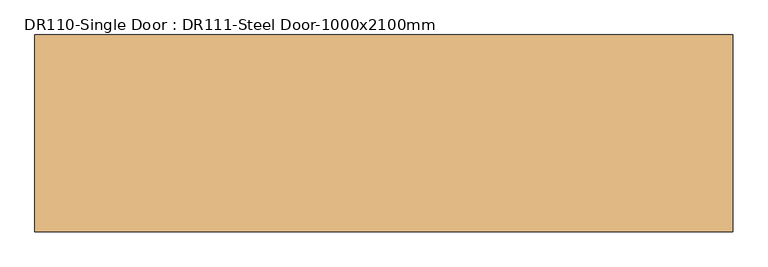
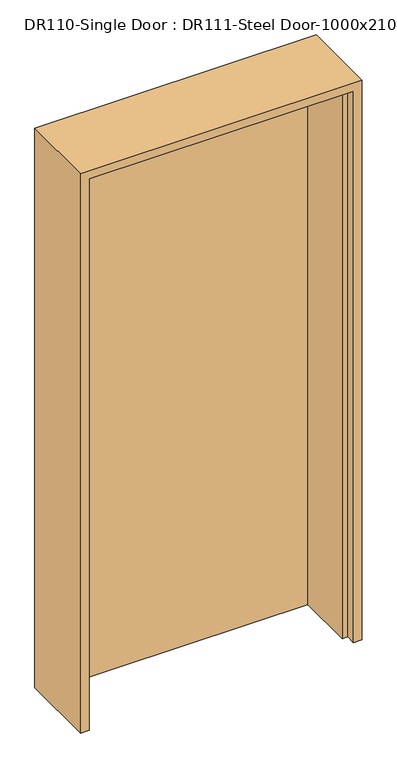
"""IFC4 building model written with IfcOpenShell, lengths in millimetres: door geometry, DR110-Single Door : DR111-Steel Door-1000x2100mm."""

import ifcopenshell
import ifcopenshell.guid

model = None  # the IFC model being written
_history = None  # IfcOwnerHistory: only IFC2X3 demands one
_inside = {}  # id of a spatial element -> (the spatial element, [elements in it])
_under = {}  # id of a project, library or spatial element -> (it, [spatial elements below it])
_declared = {}  # id of a project -> (the project, [libraries it declares])
_typed = {}  # id of a type object -> (the type object, [elements of that type])
_made_of = {}  # id of a material, layer set ... -> (it, [elements and type objects made of it])


def new_model(schema):
    """Start an empty IFC model of exactly this schema.

    Asked for "IFC4X3", IfcOpenShell would pick the latest addendum, in which some entities
    have other attributes; the version numbers below select the first issue.
    IFC2X3 requires an IfcOwnerHistory on every rooted entity: one is made here for all.
    """
    global model, _history
    if schema == "IFC4X3":
        model = ifcopenshell.file(schema_version=(4, 3, 0, 0))
    else:
        model = ifcopenshell.file(schema=schema)
    _inside.clear()
    _under.clear()
    _declared.clear()
    _typed.clear()
    _made_of.clear()
    _history = None
    if model.schema == "IFC2X3":
        org = make("IfcOrganization", Name="unknown")
        user = make(
            "IfcPersonAndOrganization",
            ThePerson=make("IfcPerson", FamilyName="unknown"),
            TheOrganization=org,
        )
        app = make(
            "IfcApplication",
            ApplicationDeveloper=org,
            Version="unknown",
            ApplicationFullName="unknown",
            ApplicationIdentifier="unknown",
        )
        _history = make(
            "IfcOwnerHistory",
            OwningUser=user,
            OwningApplication=app,
            ChangeAction="ADDED",
            CreationDate=0,
        )
    return model


def make(cls, **values):
    """One entity of the class cls with the attributes given. An attribute that is None is left unset."""
    return model.create_entity(
        cls, **{name: value for name, value in values.items() if value is not None}
    )


def rooted(cls, **values):
    """An entity with a GlobalId (a new one), such as an element, a storey or a relation."""
    return make(cls, GlobalId=ifcopenshell.guid.new(), OwnerHistory=_history, **values)


def si_unit(unit_type, name, prefix=None):
    """IfcSIUnit, for example si_unit("LENGTHUNIT", "METRE", prefix="MILLI")."""
    return make("IfcSIUnit", UnitType=unit_type, Prefix=prefix, Name=name)


def assignment(units):
    """IfcUnitAssignment: the units of a project."""
    return None if units is None else make("IfcUnitAssignment", Units=units)


def point(xyz):
    """IfcCartesianPoint."""
    return None if xyz is None else make("IfcCartesianPoint", Coordinates=xyz)


def direction(xyz):
    """IfcDirection."""
    return None if xyz is None else make("IfcDirection", DirectionRatios=xyz)


def frame(location, z_axis=None, x_axis=None):
    """IfcAxis2Placement3D, a coordinate frame: its origin and axes. An axis left out is left unset."""
    return make(
        "IfcAxis2Placement3D",
        Location=point(location),
        Axis=direction(z_axis),
        RefDirection=direction(x_axis),
    )


def origin():
    """The frame at (0, 0, 0) with its axes left unset."""
    return frame((0.0, 0.0, 0.0))


def origin_with_axes():
    """The frame at (0, 0, 0) with the z axis (0, 0, 1) and the x axis (1, 0, 0) written out."""
    return frame((0.0, 0.0, 0.0), z_axis=(0.0, 0.0, 1.0), x_axis=(1.0, 0.0, 0.0))


def place(relative_to, where):
    """IfcLocalPlacement: puts the frame where relative to a parent placement (None: the world)."""
    return make(
        "IfcLocalPlacement", PlacementRelTo=relative_to, RelativePlacement=where
    )


def context(
    kind, dimensions, precision=None, world=None, true_north=None, identifier=None
):
    """IfcGeometricRepresentationContext, for example the 3D "Model" context."""
    return make(
        "IfcGeometricRepresentationContext",
        ContextIdentifier=identifier,
        ContextType=kind,
        CoordinateSpaceDimension=dimensions,
        Precision=precision,
        WorldCoordinateSystem=world,
        TrueNorth=true_north,
    )


def project(units=None, contexts=None):
    """IfcProject with its units and contexts."""
    return rooted(
        "IfcProject",
        Name="project",
        RepresentationContexts=contexts,
        UnitsInContext=assignment(units),
    )


def spatial(cls, under=None, at=None, **own):
    """A site, building, storey or space (cls), placed at a placement, below another one or the project."""
    s = rooted(cls, ObjectPlacement=at, **own)
    if under is not None:
        _under.setdefault(under.id(), (under, []))[1].append(s)
    return s


def polyline(points):
    """IfcPolyline through the points."""
    return make("IfcPolyline", Points=[point(p) for p in points])


def outline(outer, holes=None, kind="AREA"):
    """IfcArbitraryClosedProfileDef: a profile drawn as a closed curve; with holes, ...WithVoids."""
    if holes is None:
        return make("IfcArbitraryClosedProfileDef", ProfileType=kind, OuterCurve=outer)
    return make(
        "IfcArbitraryProfileDefWithVoids",
        ProfileType=kind,
        OuterCurve=outer,
        InnerCurves=holes,
    )


def extrude(swept, where, along, depth):
    """IfcExtrudedAreaSolid: the profile swept, set in the frame where, extruded along a direction by depth."""
    return make(
        "IfcExtrudedAreaSolid",
        SweptArea=swept,
        Position=where,
        ExtrudedDirection=direction(along),
        Depth=depth,
    )


def faces_of(points, faces, orient=None, outer=None):
    """IfcFace entities. A face is a list of loops; a loop is a list of indices into points, from 0.

    orient and outer hold one flag for each loop. By default every Orientation is true, the
    first loop of a face is its IfcFaceOuterBound and the others are IfcFaceBound.
    """
    made = []
    for i, loops in enumerate(faces):
        bounds = []
        for j, loop in enumerate(loops):
            is_outer = j == 0 if outer is None else outer[i][j]
            bounds.append(
                make(
                    "IfcFaceOuterBound" if is_outer else "IfcFaceBound",
                    Bound=make("IfcPolyLoop", Polygon=[points[k] for k in loop]),
                    Orientation=True if orient is None else orient[i][j],
                )
            )
        made.append(make("IfcFace", Bounds=bounds))
    return made


def faceted_brep(points, faces, orient=None, outer=None, voids=None):
    """IfcFacetedBrep: a solid bounded by flat faces; with voids (closed shells), ...WithVoids."""
    shared = [point(p) for p in points]
    hull = make("IfcClosedShell", CfsFaces=faces_of(shared, faces, orient, outer))
    if voids is None:
        return make("IfcFacetedBrep", Outer=hull)
    return make(
        "IfcFacetedBrepWithVoids",
        Outer=hull,
        Voids=[
            make(cls, CfsFaces=faces_of(shared, fs, o, b)) for cls, fs, o, b in voids
        ],
    )


def shape(context_of_items, identifier, shape_type, items):
    """IfcShapeRepresentation: the items that make up one representation, for example the "Body"."""
    return make(
        "IfcShapeRepresentation",
        ContextOfItems=context_of_items,
        RepresentationIdentifier=identifier,
        RepresentationType=shape_type,
        Items=items,
    )


def source(mapping_origin, context_of_items, identifier, shape_type, items):
    """IfcRepresentationMap: a shape defined once, which mapped items show again and again."""
    return make(
        "IfcRepresentationMap",
        MappingOrigin=mapping_origin,
        MappedRepresentation=shape(context_of_items, identifier, shape_type, items),
    )


def transform(
    local_origin,
    x_axis=None,
    y_axis=None,
    z_axis=None,
    scale=None,
    scale2=None,
    scale3=None,
    uniform=True,
):
    """IfcCartesianTransformationOperator3D, or its non-uniform kind. x_axis, y_axis, z_axis: its Axis1, 2, 3."""
    if uniform:
        return make(
            "IfcCartesianTransformationOperator3D",
            Axis1=direction(x_axis),
            Axis2=direction(y_axis),
            LocalOrigin=point(local_origin),
            Scale=scale,
            Axis3=direction(z_axis),
        )
    return make(
        "IfcCartesianTransformationOperator3DnonUniform",
        Axis1=direction(x_axis),
        Axis2=direction(y_axis),
        LocalOrigin=point(local_origin),
        Scale=scale,
        Axis3=direction(z_axis),
        Scale2=scale2,
        Scale3=scale3,
    )


def mapped(mapping_source, mapping_target):
    """IfcMappedItem: shows the shape of a source again, moved by a transform."""
    return make(
        "IfcMappedItem", MappingSource=mapping_source, MappingTarget=mapping_target
    )


def made_of(thing, what):
    """Note that an element or type object is made of a material, layer set ...; save() writes the relation."""
    if what is not None:
        _made_of.setdefault(what.id(), (what, []))[1].append(thing)
    return thing


def element(
    cls,
    number,
    at=None,
    inside=None,
    cuts=None,
    type_object=None,
    material=None,
    context=None,
    identifier="Body",
    shape_type=None,
    held_by="IfcProductDefinitionShape",
    body=None,
    shapes=None,
    **own,
):
    """One element of the class cls, such as IfcWall. Its Tag is "e" and its number.

    at: its placement. inside: the storey or other place that contains it. cuts: it is an
    opening in that element (IfcRelVoidsElement). A single representation is given by context,
    identifier, shape_type and body (its items); several are given by shapes. held_by: the class
    of the entity that holds the representations. save() writes the other relations.
    """
    e = rooted(cls, Tag="e%d" % number, ObjectPlacement=at, **own)
    if body is not None:
        shapes = [shape(context, identifier, shape_type, body)]
    if shapes is not None:
        e.Representation = make(held_by, Representations=shapes)
    if inside is not None:
        _inside.setdefault(inside.id(), (inside, []))[1].append(e)
    if cuts is not None:
        rooted(
            "IfcRelVoidsElement", RelatingBuildingElement=cuts, RelatedOpeningElement=e
        )
    if type_object is not None:
        _typed.setdefault(type_object.id(), (type_object, []))[1].append(e)
    return made_of(e, material)


def aggregate(whole, parts):
    """IfcRelAggregates: a whole, such as a stair, and the parts it consists of."""
    return rooted("IfcRelAggregates", RelatingObject=whole, RelatedObjects=parts)


def save(model, path):
    """Write the relations noted so far, then the file.

    IfcRelAggregates (storeys below a building ...), IfcRelContainedInSpatialStructure (elements
    in a storey), IfcRelDefinesByType, IfcRelAssociatesMaterial and IfcRelDeclares: one each for
    every whole, place, type object, material and project.
    """
    for whole, parts in _under.values():
        aggregate(whole, parts)
    for where, things in _inside.values():
        rooted(
            "IfcRelContainedInSpatialStructure",
            RelatedElements=things,
            RelatingStructure=where,
        )
    for kind, things in _typed.values():
        rooted("IfcRelDefinesByType", RelatedObjects=things, RelatingType=kind)
    for what, things in _made_of.values():
        rooted("IfcRelAssociatesMaterial", RelatedObjects=things, RelatingMaterial=what)
    for by, libraries in _declared.values():
        rooted("IfcRelDeclares", RelatingContext=by, RelatedDefinitions=libraries)
    model.write(path)


def dr110_single_door_dr111_steel_door_1000x2100mm_74bb0800(model_context):
    return source(origin(), model_context, "Body", "SolidModel", [
        extrude(outline(polyline([(470.0, 141.0), (470.0, 106.0), (-470.0, 106.0), (-470.0, 141.0), (470.0, 141.0)])), origin_with_axes(), (0.0, 0.0, 1.0), 2070.0),
        faceted_brep([(470.0, 141.0, 0.0), (500.0, 141.0, 0.0), (500.0, -141.0, 0.0), (470.0, -141.0, 0.0), (470.0, -106.0, 0.0), (450.0, -106.0, 0.0), (450.0, 106.0, 0.0), (470.0, 106.0, 0.0), (470.0, 141.0, 2070.0), (-470.0, 141.0, 2070.0), (-470.0, 141.0, 0.0), (-500.0, 141.0, 0.0), (-500.0, 141.0, 2100.0), (500.0, 141.0, 2100.0), (500.0, -141.0, 2100.0), (-500.0, -141.0, 2100.0), (-500.0, -141.0, 0.0), (-470.0, -141.0, 0.0), (-470.0, -141.0, 2070.0), (470.0, -141.0, 2070.0), (470.0, -106.0, 2070.0), (-470.0, -106.0, 2070.0), (-470.0, -106.0, 0.0), (-450.0, -106.0, 0.0), (-450.0, -106.0, 2050.0), (450.0, -106.0, 2050.0), (450.0, 106.0, 2050.0), (-450.0, 106.0, 2050.0), (-450.0, 106.0, 0.0), (-470.0, 106.0, 0.0), (-470.0, 106.0, 2070.0), (470.0, 106.0, 2070.0)], [[[0, 1, 2, 3, 4, 5, 6, 7]], [[1, 0, 8, 9, 10, 11, 12, 13]], [[2, 1, 13, 14]], [[3, 2, 14, 15, 16, 17, 18, 19]], [[4, 3, 19, 20]], [[5, 4, 20, 21, 22, 23, 24, 25]], [[6, 5, 25, 26]], [[7, 6, 26, 27, 28, 29, 30, 31]], [[0, 7, 31, 8]], [[9, 30, 29, 10]], [[10, 29, 28, 23, 22, 17, 16, 11]], [[15, 12, 11, 16]], [[21, 18, 17, 22]], [[27, 24, 23, 28]], [[14, 13, 12, 15]], [[20, 19, 18, 21]], [[26, 25, 24, 27]], [[8, 31, 30, 9]]]),
    ])


if __name__ == "__main__":
    model = new_model("IFC4")
    model_context = context("Model", 3, world=origin())
    ifc_project = project(units=[si_unit("LENGTHUNIT", "METRE", prefix="MILLI")], contexts=[model_context])
    site = spatial("IfcSite", under=ifc_project)
    building = spatial("IfcBuilding", under=site)
    placement = place(None, origin())
    dr110_single_door_dr111_steel_door_1000x2100mm_shape = dr110_single_door_dr111_steel_door_1000x2100mm_74bb0800(model_context)
    element("IfcDoor", 1, ObjectType="DR110-Single Door : DR111-Steel Door-1000x2100mm", at=placement, inside=building, context=model_context, shape_type="MappedRepresentation", body=[
        mapped(dr110_single_door_dr111_steel_door_1000x2100mm_shape, transform((0.0, 0.0, 0.0), x_axis=(1.0, 0.0, 0.0), y_axis=(0.0, 1.0, 0.0), z_axis=(0.0, 0.0, 1.0))),
    ])
    save(model, "model.ifc")

# Revit data of these elements
# Type "DR110-Single Door : DR111-Steel Door-1000x2100mm"
#   Description = "DSDSSD"
#   Type Mark = "SD"
#   Analytic Construction = "<None>"
#   프레임 투영 외부. = 25 mm
#   프레임 투영 내부. = 25 mm
#   프레임 폭 = 75 mm
#   Height = 2100 mm
#   Width = 1000 mm
#   Define Thermal Properties by = 1
#   문 패널 = SD1 문 패널
#   문 프레임 = A04AQ098-00002_Steel Door_non FP_single
#   Function = (empty or 0)
#   Wall Closure = (empty or 0)
# Element 1 (IfcDoor, "DR110-Single Door : DR111-Steel Door-1000x2100mm")
#   Materials on its faces: "A04AQ098-00002_Steel Door_non FP_single", "SD1 문 패널"
# Materials
#   "SD1 문 패널": class "금속", colour RGB 247 247 247, transparency 0, Description = "STEEL DOOR (1000Wx2100H)"
#   "A04AQ098-00002_Steel Door_non FP_single": class "금속", colour RGB 247 247 247, transparency 0, Description = "Steel Door", W00) Work Master Code = "A04AQ098-00002", W01) Work Master_Lv1 = "Finishing Work", W02) Work Master_Lv2 = "Door & Window Work", W03) Work Master_Spec.1 = "Steel Door w/ Steel Frame", W04) Work Master_Spec.2 = "Fire Protective Rating: N/A, Single Door", W05) Work Master_Spec.3 = "w/ Hardware & Accessories", Cost = 0
